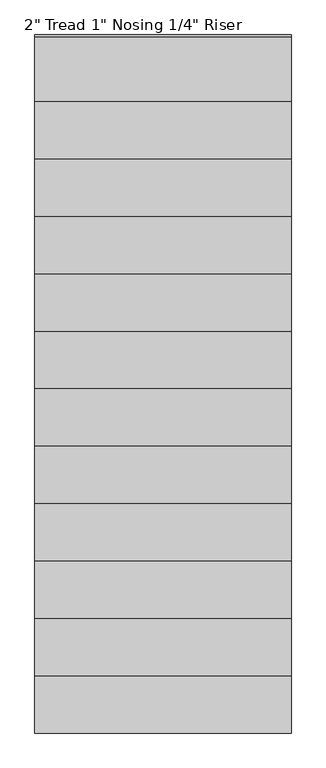
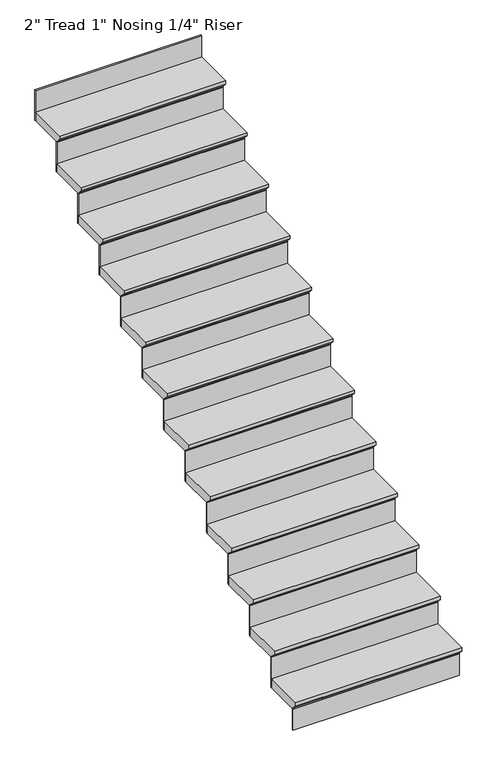
"""IFC4 building model written with IfcOpenShell, lengths in millimetres: stair flight geometry."""

import ifcopenshell
import ifcopenshell.guid

model = None  # the IFC model being written
_history = None  # IfcOwnerHistory: only IFC2X3 demands one
_inside = {}  # id of a spatial element -> (the spatial element, [elements in it])
_under = {}  # id of a project, library or spatial element -> (it, [spatial elements below it])
_declared = {}  # id of a project -> (the project, [libraries it declares])
_typed = {}  # id of a type object -> (the type object, [elements of that type])
_made_of = {}  # id of a material, layer set ... -> (it, [elements and type objects made of it])


def new_model(schema):
    """Start an empty IFC model of exactly this schema.

    Asked for "IFC4X3", IfcOpenShell would pick the latest addendum, in which some entities
    have other attributes; the version numbers below select the first issue.
    IFC2X3 requires an IfcOwnerHistory on every rooted entity: one is made here for all.
    """
    global model, _history
    if schema == "IFC4X3":
        model = ifcopenshell.file(schema_version=(4, 3, 0, 0))
    else:
        model = ifcopenshell.file(schema=schema)
    _inside.clear()
    _under.clear()
    _declared.clear()
    _typed.clear()
    _made_of.clear()
    _history = None
    if model.schema == "IFC2X3":
        org = make("IfcOrganization", Name="unknown")
        user = make(
            "IfcPersonAndOrganization",
            ThePerson=make("IfcPerson", FamilyName="unknown"),
            TheOrganization=org,
        )
        app = make(
            "IfcApplication",
            ApplicationDeveloper=org,
            Version="unknown",
            ApplicationFullName="unknown",
            ApplicationIdentifier="unknown",
        )
        _history = make(
            "IfcOwnerHistory",
            OwningUser=user,
            OwningApplication=app,
            ChangeAction="ADDED",
            CreationDate=0,
        )
    return model


def make(cls, **values):
    """One entity of the class cls with the attributes given. An attribute that is None is left unset."""
    return model.create_entity(
        cls, **{name: value for name, value in values.items() if value is not None}
    )


def rooted(cls, **values):
    """An entity with a GlobalId (a new one), such as an element, a storey or a relation."""
    return make(cls, GlobalId=ifcopenshell.guid.new(), OwnerHistory=_history, **values)


def si_unit(unit_type, name, prefix=None):
    """IfcSIUnit, for example si_unit("LENGTHUNIT", "METRE", prefix="MILLI")."""
    return make("IfcSIUnit", UnitType=unit_type, Prefix=prefix, Name=name)


def assignment(units):
    """IfcUnitAssignment: the units of a project."""
    return None if units is None else make("IfcUnitAssignment", Units=units)


def point(xyz):
    """IfcCartesianPoint."""
    return None if xyz is None else make("IfcCartesianPoint", Coordinates=xyz)


def direction(xyz):
    """IfcDirection."""
    return None if xyz is None else make("IfcDirection", DirectionRatios=xyz)


def frame(location, z_axis=None, x_axis=None):
    """IfcAxis2Placement3D, a coordinate frame: its origin and axes. An axis left out is left unset."""
    return make(
        "IfcAxis2Placement3D",
        Location=point(location),
        Axis=direction(z_axis),
        RefDirection=direction(x_axis),
    )


def origin():
    """The frame at (0, 0, 0) with its axes left unset."""
    return frame((0.0, 0.0, 0.0))


def place(relative_to, where):
    """IfcLocalPlacement: puts the frame where relative to a parent placement (None: the world)."""
    return make(
        "IfcLocalPlacement", PlacementRelTo=relative_to, RelativePlacement=where
    )


def context(
    kind, dimensions, precision=None, world=None, true_north=None, identifier=None
):
    """IfcGeometricRepresentationContext, for example the 3D "Model" context."""
    return make(
        "IfcGeometricRepresentationContext",
        ContextIdentifier=identifier,
        ContextType=kind,
        CoordinateSpaceDimension=dimensions,
        Precision=precision,
        WorldCoordinateSystem=world,
        TrueNorth=true_north,
    )


def project(units=None, contexts=None):
    """IfcProject with its units and contexts."""
    return rooted(
        "IfcProject",
        Name="project",
        RepresentationContexts=contexts,
        UnitsInContext=assignment(units),
    )


def spatial(cls, under=None, at=None, **own):
    """A site, building, storey or space (cls), placed at a placement, below another one or the project."""
    s = rooted(cls, ObjectPlacement=at, **own)
    if under is not None:
        _under.setdefault(under.id(), (under, []))[1].append(s)
    return s


def polyline(points):
    """IfcPolyline through the points."""
    return make("IfcPolyline", Points=[point(p) for p in points])


def outline(outer, holes=None, kind="AREA"):
    """IfcArbitraryClosedProfileDef: a profile drawn as a closed curve; with holes, ...WithVoids."""
    if holes is None:
        return make("IfcArbitraryClosedProfileDef", ProfileType=kind, OuterCurve=outer)
    return make(
        "IfcArbitraryProfileDefWithVoids",
        ProfileType=kind,
        OuterCurve=outer,
        InnerCurves=holes,
    )


def extrude(swept, where, along, depth):
    """IfcExtrudedAreaSolid: the profile swept, set in the frame where, extruded along a direction by depth."""
    return make(
        "IfcExtrudedAreaSolid",
        SweptArea=swept,
        Position=where,
        ExtrudedDirection=direction(along),
        Depth=depth,
    )


def shape(context_of_items, identifier, shape_type, items):
    """IfcShapeRepresentation: the items that make up one representation, for example the "Body"."""
    return make(
        "IfcShapeRepresentation",
        ContextOfItems=context_of_items,
        RepresentationIdentifier=identifier,
        RepresentationType=shape_type,
        Items=items,
    )


def source(mapping_origin, context_of_items, identifier, shape_type, items):
    """IfcRepresentationMap: a shape defined once, which mapped items show again and again."""
    return make(
        "IfcRepresentationMap",
        MappingOrigin=mapping_origin,
        MappedRepresentation=shape(context_of_items, identifier, shape_type, items),
    )


def transform(
    local_origin,
    x_axis=None,
    y_axis=None,
    z_axis=None,
    scale=None,
    scale2=None,
    scale3=None,
    uniform=True,
):
    """IfcCartesianTransformationOperator3D, or its non-uniform kind. x_axis, y_axis, z_axis: its Axis1, 2, 3."""
    if uniform:
        return make(
            "IfcCartesianTransformationOperator3D",
            Axis1=direction(x_axis),
            Axis2=direction(y_axis),
            LocalOrigin=point(local_origin),
            Scale=scale,
            Axis3=direction(z_axis),
        )
    return make(
        "IfcCartesianTransformationOperator3DnonUniform",
        Axis1=direction(x_axis),
        Axis2=direction(y_axis),
        LocalOrigin=point(local_origin),
        Scale=scale,
        Axis3=direction(z_axis),
        Scale2=scale2,
        Scale3=scale3,
    )


def mapped(mapping_source, mapping_target):
    """IfcMappedItem: shows the shape of a source again, moved by a transform."""
    return make(
        "IfcMappedItem", MappingSource=mapping_source, MappingTarget=mapping_target
    )


def made_of(thing, what):
    """Note that an element or type object is made of a material, layer set ...; save() writes the relation."""
    if what is not None:
        _made_of.setdefault(what.id(), (what, []))[1].append(thing)
    return thing


def element(
    cls,
    number,
    at=None,
    inside=None,
    cuts=None,
    type_object=None,
    material=None,
    context=None,
    identifier="Body",
    shape_type=None,
    held_by="IfcProductDefinitionShape",
    body=None,
    shapes=None,
    **own,
):
    """One element of the class cls, such as IfcWall. Its Tag is "e" and its number.

    at: its placement. inside: the storey or other place that contains it. cuts: it is an
    opening in that element (IfcRelVoidsElement). A single representation is given by context,
    identifier, shape_type and body (its items); several are given by shapes. held_by: the class
    of the entity that holds the representations. save() writes the other relations.
    """
    e = rooted(cls, Tag="e%d" % number, ObjectPlacement=at, **own)
    if body is not None:
        shapes = [shape(context, identifier, shape_type, body)]
    if shapes is not None:
        e.Representation = make(held_by, Representations=shapes)
    if inside is not None:
        _inside.setdefault(inside.id(), (inside, []))[1].append(e)
    if cuts is not None:
        rooted(
            "IfcRelVoidsElement", RelatingBuildingElement=cuts, RelatedOpeningElement=e
        )
    if type_object is not None:
        _typed.setdefault(type_object.id(), (type_object, []))[1].append(e)
    return made_of(e, material)


def aggregate(whole, parts):
    """IfcRelAggregates: a whole, such as a stair, and the parts it consists of."""
    return rooted("IfcRelAggregates", RelatingObject=whole, RelatedObjects=parts)


def save(model, path):
    """Write the relations noted so far, then the file.

    IfcRelAggregates (storeys below a building ...), IfcRelContainedInSpatialStructure (elements
    in a storey), IfcRelDefinesByType, IfcRelAssociatesMaterial and IfcRelDeclares: one each for
    every whole, place, type object, material and project.
    """
    for whole, parts in _under.values():
        aggregate(whole, parts)
    for where, things in _inside.values():
        rooted(
            "IfcRelContainedInSpatialStructure",
            RelatedElements=things,
            RelatingStructure=where,
        )
    for kind, things in _typed.values():
        rooted("IfcRelDefinesByType", RelatedObjects=things, RelatingType=kind)
    for what, things in _made_of.values():
        rooted("IfcRelAssociatesMaterial", RelatedObjects=things, RelatingMaterial=what)
    for by, libraries in _declared.values():
        rooted("IfcRelDeclares", RelatingContext=by, RelatedDefinitions=libraries)
    model.write(path)


def stair_flight_443dce11(model_context):
    return source(origin(), model_context, "Body", "SweptSolid", [
        extrude(outline(polyline([(-12572.2570712, -2092.5692308), (-12343.6570712, -2092.5692308), (-12343.6570712, -2143.3692308), (-12546.8570712, -2143.3692308), (-12546.8570712, -2137.0192308), (-12572.2570712, -2111.6192308), (-12572.2570712, -2092.5692308)])), frame((-25042.4664763, 0.0, 0.0), z_axis=(1.0, 0.0, 0.0), x_axis=(0.0, 1.0, 0.0)), (0.0, 0.0, 1.0), 908.05),
        extrude(outline(polyline([(-24134.4164763, -12540.5070712), (-24134.4164763, -12546.8570712), (-25042.4664763, -12546.8570712), (-25042.4664763, -12540.5070712), (-24134.4164763, -12540.5070712)])), frame((0.0, 0.0, -2266.95), z_axis=(0.0, 0.0, 1.0), x_axis=(1.0, 0.0, 0.0)), (0.0, 0.0, 1.0), 123.5807692),
        extrude(outline(polyline([(-24134.4164763, -12337.3070712), (-24134.4164763, -12343.6570712), (-25042.4664763, -12343.6570712), (-25042.4664763, -12337.3070712), (-24134.4164763, -12337.3070712)])), frame((0.0, 0.0, -2143.3692308), z_axis=(0.0, 0.0, 1.0), x_axis=(1.0, 0.0, 0.0)), (0.0, 0.0, 1.0), 174.3807692),
        extrude(outline(polyline([(-12369.0570712, -1918.1884615), (-12140.4570712, -1918.1884615), (-12140.4570712, -1968.9884615), (-12343.6570712, -1968.9884615), (-12343.6570712, -1962.6384615), (-12369.0570712, -1937.2384615), (-12369.0570712, -1918.1884615)])), frame((-25042.4664763, 0.0, 0.0), z_axis=(1.0, 0.0, 0.0), x_axis=(0.0, 1.0, 0.0)), (0.0, 0.0, 1.0), 908.05),
        extrude(outline(polyline([(-24134.4164763, -12134.1070712), (-24134.4164763, -12140.4570712), (-25042.4664763, -12140.4570712), (-25042.4664763, -12134.1070712), (-24134.4164763, -12134.1070712)])), frame((0.0, 0.0, -1968.9884615), z_axis=(0.0, 0.0, 1.0), x_axis=(1.0, 0.0, 0.0)), (0.0, 0.0, 1.0), 174.3807692),
        extrude(outline(polyline([(-12165.8570712, -1743.8076923), (-11937.2570712, -1743.8076923), (-11937.2570712, -1794.6076923), (-12140.4570712, -1794.6076923), (-12140.4570712, -1788.2576923), (-12165.8570712, -1762.8576923), (-12165.8570712, -1743.8076923)])), frame((-25042.4664763, 0.0, 0.0), z_axis=(1.0, 0.0, 0.0), x_axis=(0.0, 1.0, 0.0)), (0.0, 0.0, 1.0), 908.05),
        extrude(outline(polyline([(-24134.4164763, -11930.9070712), (-24134.4164763, -11937.2570712), (-25042.4664763, -11937.2570712), (-25042.4664763, -11930.9070712), (-24134.4164763, -11930.9070712)])), frame((0.0, 0.0, -1794.6076923), z_axis=(0.0, 0.0, 1.0), x_axis=(1.0, 0.0, 0.0)), (0.0, 0.0, 1.0), 174.3807692),
        extrude(outline(polyline([(-11962.6570712, -1569.4269231), (-11734.0570712, -1569.4269231), (-11734.0570712, -1620.2269231), (-11937.2570712, -1620.2269231), (-11937.2570712, -1613.8769231), (-11962.6570712, -1588.4769231), (-11962.6570712, -1569.4269231)])), frame((-25042.4664763, 0.0, 0.0), z_axis=(1.0, 0.0, 0.0), x_axis=(0.0, 1.0, 0.0)), (0.0, 0.0, 1.0), 908.05),
        extrude(outline(polyline([(-24134.4164763, -11727.7070712), (-24134.4164763, -11734.0570712), (-25042.4664763, -11734.0570712), (-25042.4664763, -11727.7070712), (-24134.4164763, -11727.7070712)])), frame((0.0, 0.0, -1620.2269231), z_axis=(0.0, 0.0, 1.0), x_axis=(1.0, 0.0, 0.0)), (0.0, 0.0, 1.0), 174.3807692),
        extrude(outline(polyline([(-11759.4570712, -1395.0461538), (-11530.8570712, -1395.0461538), (-11530.8570712, -1445.8461538), (-11734.0570712, -1445.8461538), (-11734.0570712, -1439.4961538), (-11759.4570712, -1414.0961538), (-11759.4570712, -1395.0461538)])), frame((-25042.4664763, 0.0, 0.0), z_axis=(1.0, 0.0, 0.0), x_axis=(0.0, 1.0, 0.0)), (0.0, 0.0, 1.0), 908.05),
        extrude(outline(polyline([(-24134.4164763, -11524.5070712), (-24134.4164763, -11530.8570712), (-25042.4664763, -11530.8570712), (-25042.4664763, -11524.5070712), (-24134.4164763, -11524.5070712)])), frame((0.0, 0.0, -1445.8461538), z_axis=(0.0, 0.0, 1.0), x_axis=(1.0, 0.0, 0.0)), (0.0, 0.0, 1.0), 174.3807692),
        extrude(outline(polyline([(-11556.2570712, -1220.6653846), (-11327.6570712, -1220.6653846), (-11327.6570712, -1271.4653846), (-11530.8570712, -1271.4653846), (-11530.8570712, -1265.1153846), (-11556.2570712, -1239.7153846), (-11556.2570712, -1220.6653846)])), frame((-25042.4664763, 0.0, 0.0), z_axis=(1.0, 0.0, 0.0), x_axis=(0.0, 1.0, 0.0)), (0.0, 0.0, 1.0), 908.05),
        extrude(outline(polyline([(-24134.4164763, -11321.3070712), (-24134.4164763, -11327.6570712), (-25042.4664763, -11327.6570712), (-25042.4664763, -11321.3070712), (-24134.4164763, -11321.3070712)])), frame((0.0, 0.0, -1271.4653846), z_axis=(0.0, 0.0, 1.0), x_axis=(1.0, 0.0, 0.0)), (0.0, 0.0, 1.0), 174.3807692),
        extrude(outline(polyline([(-11353.0570712, -1046.2846154), (-11124.4570712, -1046.2846154), (-11124.4570712, -1097.0846154), (-11327.6570712, -1097.0846154), (-11327.6570712, -1090.7346154), (-11353.0570712, -1065.3346154), (-11353.0570712, -1046.2846154)])), frame((-25042.4664763, 0.0, 0.0), z_axis=(1.0, 0.0, 0.0), x_axis=(0.0, 1.0, 0.0)), (0.0, 0.0, 1.0), 908.05),
        extrude(outline(polyline([(-24134.4164763, -11118.1070712), (-24134.4164763, -11124.4570712), (-25042.4664763, -11124.4570712), (-25042.4664763, -11118.1070712), (-24134.4164763, -11118.1070712)])), frame((0.0, 0.0, -1097.0846154), z_axis=(0.0, 0.0, 1.0), x_axis=(1.0, 0.0, 0.0)), (0.0, 0.0, 1.0), 174.3807692),
        extrude(outline(polyline([(-11149.8570712, -871.9038462), (-10921.2570712, -871.9038462), (-10921.2570712, -922.7038462), (-11124.4570712, -922.7038462), (-11124.4570712, -916.3538462), (-11149.8570712, -890.9538462), (-11149.8570712, -871.9038462)])), frame((-25042.4664763, 0.0, 0.0), z_axis=(1.0, 0.0, 0.0), x_axis=(0.0, 1.0, 0.0)), (0.0, 0.0, 1.0), 908.05),
        extrude(outline(polyline([(-24134.4164763, -10914.9070712), (-24134.4164763, -10921.2570712), (-25042.4664763, -10921.2570712), (-25042.4664763, -10914.9070712), (-24134.4164763, -10914.9070712)])), frame((0.0, 0.0, -922.7038462), z_axis=(0.0, 0.0, 1.0), x_axis=(1.0, 0.0, 0.0)), (0.0, 0.0, 1.0), 174.3807692),
        extrude(outline(polyline([(-10946.6570712, -697.5230769), (-10718.0570712, -697.5230769), (-10718.0570712, -748.3230769), (-10921.2570712, -748.3230769), (-10921.2570712, -741.9730769), (-10946.6570712, -716.5730769), (-10946.6570712, -697.5230769)])), frame((-25042.4664763, 0.0, 0.0), z_axis=(1.0, 0.0, 0.0), x_axis=(0.0, 1.0, 0.0)), (0.0, 0.0, 1.0), 908.05),
        extrude(outline(polyline([(-24134.4164763, -10711.7070712), (-24134.4164763, -10718.0570712), (-25042.4664763, -10718.0570712), (-25042.4664763, -10711.7070712), (-24134.4164763, -10711.7070712)])), frame((0.0, 0.0, -748.3230769), z_axis=(0.0, 0.0, 1.0), x_axis=(1.0, 0.0, 0.0)), (0.0, 0.0, 1.0), 174.3807692),
        extrude(outline(polyline([(-10743.4570712, -523.1423077), (-10514.8570712, -523.1423077), (-10514.8570712, -573.9423077), (-10718.0570712, -573.9423077), (-10718.0570712, -567.5923077), (-10743.4570712, -542.1923077), (-10743.4570712, -523.1423077)])), frame((-25042.4664763, 0.0, 0.0), z_axis=(1.0, 0.0, 0.0), x_axis=(0.0, 1.0, 0.0)), (0.0, 0.0, 1.0), 908.05),
        extrude(outline(polyline([(-24134.4164763, -10508.5070712), (-24134.4164763, -10514.8570712), (-25042.4664763, -10514.8570712), (-25042.4664763, -10508.5070712), (-24134.4164763, -10508.5070712)])), frame((0.0, 0.0, -573.9423077), z_axis=(0.0, 0.0, 1.0), x_axis=(1.0, 0.0, 0.0)), (0.0, 0.0, 1.0), 174.3807692),
        extrude(outline(polyline([(-10540.2570712, -348.7615385), (-10311.6570712, -348.7615385), (-10311.6570712, -399.5615385), (-10514.8570712, -399.5615385), (-10514.8570712, -393.2115385), (-10540.2570712, -367.8115385), (-10540.2570712, -348.7615385)])), frame((-25042.4664763, 0.0, 0.0), z_axis=(1.0, 0.0, 0.0), x_axis=(0.0, 1.0, 0.0)), (0.0, 0.0, 1.0), 908.05),
        extrude(outline(polyline([(-24134.4164763, -10305.3070712), (-24134.4164763, -10311.6570712), (-25042.4664763, -10311.6570712), (-25042.4664763, -10305.3070712), (-24134.4164763, -10305.3070712)])), frame((0.0, 0.0, -399.5615385), z_axis=(0.0, 0.0, 1.0), x_axis=(1.0, 0.0, 0.0)), (0.0, 0.0, 1.0), 174.3807692),
        extrude(outline(polyline([(-24134.4164763, -10102.1070712), (-24134.4164763, -10108.4570712), (-25042.4664763, -10108.4570712), (-25042.4664763, -10102.1070712), (-24134.4164763, -10102.1070712)])), frame((0.0, 0.0, -225.1807692), z_axis=(0.0, 0.0, 1.0), x_axis=(1.0, 0.0, 0.0)), (0.0, 0.0, 1.0), 174.3807692),
        extrude(outline(polyline([(-10337.0570712, -174.3807692), (-10108.4570712, -174.3807692), (-10108.4570712, -225.1807692), (-10311.6570712, -225.1807692), (-10311.6570712, -218.8307692), (-10337.0570712, -193.4307692), (-10337.0570712, -174.3807692)])), frame((-25042.4664763, 0.0, 0.0), z_axis=(1.0, 0.0, 0.0), x_axis=(0.0, 1.0, 0.0)), (0.0, 0.0, 1.0), 908.05),
    ])


if __name__ == "__main__":
    model = new_model("IFC4")
    model_context = context("Model", 3, world=origin())
    ifc_project = project(units=[si_unit("LENGTHUNIT", "METRE", prefix="MILLI")], contexts=[model_context])
    site = spatial("IfcSite", under=ifc_project)
    building = spatial("IfcBuilding", under=site)
    placement = place(None, origin())
    stair_flight_shape = stair_flight_443dce11(model_context)
    element("IfcStairFlight", 1, ObjectType="2\" Tread 1\" Nosing 1/4\" Riser", at=placement, inside=building, context=model_context, shape_type="MappedRepresentation", body=[
        mapped(stair_flight_shape, transform((0.0, 0.0, 0.0), x_axis=(1.0, 0.0, 0.0), y_axis=(0.0, 1.0, 0.0), z_axis=(0.0, 0.0, 1.0))),
    ])
    save(model, "model.ifc")
